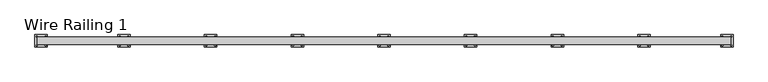
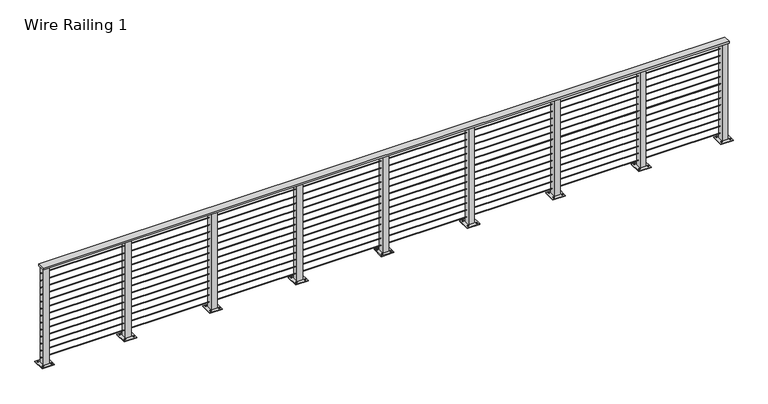
"""IFC4 building model written with IfcOpenShell, lengths in millimetres: railing geometry, Wire Railing 1."""

from ifc_helpers import new_model, si_unit, point, frame, frame_2d, origin, place, context, project, spatial, polyline, circle_curve, trimmed, segment, composite_curve, outline, extrude, source, transform, mapped, element, save


def wire_railing_1_4a66abef(model_context):
    return source(origin(), model_context, "Body", "SweptSolid", [
        extrude(outline(polyline([(-9024.2668771, -3185.4818735), (-9024.2668771, -3109.2818735), (-2001.1668771, -3109.2818735), (-2001.1668771, -3185.4818735), (-9024.2668771, -3185.4818735)])), frame((0.0, 0.0, 4502.15), z_axis=(0.0, 0.0, 1.0), x_axis=(1.0, 0.0, 0.0)), (0.0, 0.0, 1.0), 19.05),
        extrude(outline(composite_curve([segment(trimmed(circle_curve(frame_2d((-3147.3818735, 4442.61875)), 2.38125), [point((-3149.7631235, 4442.61875))], [point((-3145.0006235, 4442.61875))], False, "CARTESIAN"), True, "CONTINUOUS"), segment(trimmed(circle_curve(frame_2d((-3147.3818735, 4442.61875)), 2.38125), [point((-3145.0006235, 4442.61875))], [point((-3149.7631235, 4442.61875))], False, "CARTESIAN"), True, "CONTINUOUS")], self_intersect=False)), frame((-9024.2668771, 0.0, 0.0), z_axis=(1.0, 0.0, 0.0), x_axis=(0.0, 1.0, 0.0)), (0.0, 0.0, 1.0), 7023.1),
        extrude(outline(composite_curve([segment(trimmed(circle_curve(frame_2d((-3147.3818735, 4366.41875)), 2.38125), [point((-3149.7631235, 4366.41875))], [point((-3145.0006235, 4366.41875))], False, "CARTESIAN"), True, "CONTINUOUS"), segment(trimmed(circle_curve(frame_2d((-3147.3818735, 4366.41875)), 2.38125), [point((-3145.0006235, 4366.41875))], [point((-3149.7631235, 4366.41875))], False, "CARTESIAN"), True, "CONTINUOUS")], self_intersect=False)), frame((-9024.2668771, 0.0, 0.0), z_axis=(1.0, 0.0, 0.0), x_axis=(0.0, 1.0, 0.0)), (0.0, 0.0, 1.0), 7023.1),
        extrude(outline(composite_curve([segment(trimmed(circle_curve(frame_2d((-3147.3818735, 4290.21875)), 2.38125), [point((-3149.7631235, 4290.21875))], [point((-3145.0006235, 4290.21875))], False, "CARTESIAN"), True, "CONTINUOUS"), segment(trimmed(circle_curve(frame_2d((-3147.3818735, 4290.21875)), 2.38125), [point((-3145.0006235, 4290.21875))], [point((-3149.7631235, 4290.21875))], False, "CARTESIAN"), True, "CONTINUOUS")], self_intersect=False)), frame((-9024.2668771, 0.0, 0.0), z_axis=(1.0, 0.0, 0.0), x_axis=(0.0, 1.0, 0.0)), (0.0, 0.0, 1.0), 7023.1),
        extrude(outline(composite_curve([segment(trimmed(circle_curve(frame_2d((-3147.3818735, 4214.01875)), 2.38125), [point((-3149.7631235, 4214.01875))], [point((-3145.0006235, 4214.01875))], False, "CARTESIAN"), True, "CONTINUOUS"), segment(trimmed(circle_curve(frame_2d((-3147.3818735, 4214.01875)), 2.38125), [point((-3145.0006235, 4214.01875))], [point((-3149.7631235, 4214.01875))], False, "CARTESIAN"), True, "CONTINUOUS")], self_intersect=False)), frame((-9024.2668771, 0.0, 0.0), z_axis=(1.0, 0.0, 0.0), x_axis=(0.0, 1.0, 0.0)), (0.0, 0.0, 1.0), 7023.1),
        extrude(outline(composite_curve([segment(trimmed(circle_curve(frame_2d((-3147.3818735, 4137.81875)), 2.38125), [point((-3149.7631235, 4137.81875))], [point((-3145.0006235, 4137.81875))], False, "CARTESIAN"), True, "CONTINUOUS"), segment(trimmed(circle_curve(frame_2d((-3147.3818735, 4137.81875)), 2.38125), [point((-3145.0006235, 4137.81875))], [point((-3149.7631235, 4137.81875))], False, "CARTESIAN"), True, "CONTINUOUS")], self_intersect=False)), frame((-9024.2668771, 0.0, 0.0), z_axis=(1.0, 0.0, 0.0), x_axis=(0.0, 1.0, 0.0)), (0.0, 0.0, 1.0), 7023.1),
        extrude(outline(composite_curve([segment(trimmed(circle_curve(frame_2d((-3147.3818735, 4061.61875)), 2.38125), [point((-3149.7631235, 4061.61875))], [point((-3145.0006235, 4061.61875))], False, "CARTESIAN"), True, "CONTINUOUS"), segment(trimmed(circle_curve(frame_2d((-3147.3818735, 4061.61875)), 2.38125), [point((-3145.0006235, 4061.61875))], [point((-3149.7631235, 4061.61875))], False, "CARTESIAN"), True, "CONTINUOUS")], self_intersect=False)), frame((-9024.2668771, 0.0, 0.0), z_axis=(1.0, 0.0, 0.0), x_axis=(0.0, 1.0, 0.0)), (0.0, 0.0, 1.0), 7023.1),
        extrude(outline(composite_curve([segment(trimmed(circle_curve(frame_2d((-3147.3818735, 3985.41875)), 2.38125), [point((-3149.7631235, 3985.41875))], [point((-3145.0006235, 3985.41875))], False, "CARTESIAN"), True, "CONTINUOUS"), segment(trimmed(circle_curve(frame_2d((-3147.3818735, 3985.41875)), 2.38125), [point((-3145.0006235, 3985.41875))], [point((-3149.7631235, 3985.41875))], False, "CARTESIAN"), True, "CONTINUOUS")], self_intersect=False)), frame((-9024.2668771, 0.0, 0.0), z_axis=(1.0, 0.0, 0.0), x_axis=(0.0, 1.0, 0.0)), (0.0, 0.0, 1.0), 7023.1),
        extrude(outline(composite_curve([segment(trimmed(circle_curve(frame_2d((-3147.3818735, 3909.21875)), 2.38125), [point((-3149.7631235, 3909.21875))], [point((-3145.0006235, 3909.21875))], False, "CARTESIAN"), True, "CONTINUOUS"), segment(trimmed(circle_curve(frame_2d((-3147.3818735, 3909.21875)), 2.38125), [point((-3145.0006235, 3909.21875))], [point((-3149.7631235, 3909.21875))], False, "CARTESIAN"), True, "CONTINUOUS")], self_intersect=False)), frame((-9024.2668771, 0.0, 0.0), z_axis=(1.0, 0.0, 0.0), x_axis=(0.0, 1.0, 0.0)), (0.0, 0.0, 1.0), 7023.1),
        extrude(outline(composite_curve([segment(trimmed(circle_curve(frame_2d((-3147.3818735, 3833.01875)), 2.38125), [point((-3149.7631235, 3833.01875))], [point((-3145.0006235, 3833.01875))], False, "CARTESIAN"), True, "CONTINUOUS"), segment(trimmed(circle_curve(frame_2d((-3147.3818735, 3833.01875)), 2.38125), [point((-3145.0006235, 3833.01875))], [point((-3149.7631235, 3833.01875))], False, "CARTESIAN"), True, "CONTINUOUS")], self_intersect=False)), frame((-9024.2668771, 0.0, 0.0), z_axis=(1.0, 0.0, 0.0), x_axis=(0.0, 1.0, 0.0)), (0.0, 0.0, 1.0), 7023.1),
        extrude(outline(composite_curve([segment(trimmed(circle_curve(frame_2d((-3147.3818735, 3756.81875)), 2.38125), [point((-3149.7631235, 3756.81875))], [point((-3145.0006235, 3756.81875))], False, "CARTESIAN"), True, "CONTINUOUS"), segment(trimmed(circle_curve(frame_2d((-3147.3818735, 3756.81875)), 2.38125), [point((-3145.0006235, 3756.81875))], [point((-3149.7631235, 3756.81875))], False, "CARTESIAN"), True, "CONTINUOUS")], self_intersect=False)), frame((-9024.2668771, 0.0, 0.0), z_axis=(1.0, 0.0, 0.0), x_axis=(0.0, 1.0, 0.0)), (0.0, 0.0, 1.0), 7023.1),
        extrude(outline(composite_curve([segment(trimmed(circle_curve(frame_2d((-3147.3818735, 3680.61875)), 2.38125), [point((-3149.7631235, 3680.61875))], [point((-3145.0006235, 3680.61875))], False, "CARTESIAN"), True, "CONTINUOUS"), segment(trimmed(circle_curve(frame_2d((-3147.3818735, 3680.61875)), 2.38125), [point((-3145.0006235, 3680.61875))], [point((-3149.7631235, 3680.61875))], False, "CARTESIAN"), True, "CONTINUOUS")], self_intersect=False)), frame((-9024.2668771, 0.0, 0.0), z_axis=(1.0, 0.0, 0.0), x_axis=(0.0, 1.0, 0.0)), (0.0, 0.0, 1.0), 7023.1),
        extrude(outline(composite_curve([segment(trimmed(circle_curve(frame_2d((-3147.3818735, 3604.41875)), 2.38125), [point((-3149.7631235, 3604.41875))], [point((-3145.0006235, 3604.41875))], False, "CARTESIAN"), True, "CONTINUOUS"), segment(trimmed(circle_curve(frame_2d((-3147.3818735, 3604.41875)), 2.38125), [point((-3145.0006235, 3604.41875))], [point((-3149.7631235, 3604.41875))], False, "CARTESIAN"), True, "CONTINUOUS")], self_intersect=False)), frame((-9024.2668771, 0.0, 0.0), z_axis=(1.0, 0.0, 0.0), x_axis=(0.0, 1.0, 0.0)), (0.0, 0.0, 1.0), 7023.1),
        extrude(outline(composite_curve([segment(trimmed(circle_curve(frame_2d((-3147.3818735, 3528.21875)), 2.38125), [point((-3149.7631235, 3528.21875))], [point((-3145.0006235, 3528.21875))], False, "CARTESIAN"), True, "CONTINUOUS"), segment(trimmed(circle_curve(frame_2d((-3147.3818735, 3528.21875)), 2.38125), [point((-3145.0006235, 3528.21875))], [point((-3149.7631235, 3528.21875))], False, "CARTESIAN"), True, "CONTINUOUS")], self_intersect=False)), frame((-9024.2668771, 0.0, 0.0), z_axis=(1.0, 0.0, 0.0), x_axis=(0.0, 1.0, 0.0)), (0.0, 0.0, 1.0), 7023.1),
        extrude(outline(composite_curve([segment(trimmed(circle_curve(frame_2d((-2923.5043771, -3102.9318735)), 6.35), [point((-2923.5043771, -3096.5818735))], [point((-2923.5043771, -3109.2818735))], False, "CARTESIAN"), True, "CONTINUOUS"), segment(trimmed(circle_curve(frame_2d((-2923.5043771, -3102.9318735)), 6.35), [point((-2923.5043771, -3109.2818735))], [point((-2923.5043771, -3096.5818735))], False, "CARTESIAN"), True, "CONTINUOUS")], self_intersect=False)), frame((0.0, 0.0, 3454.4), z_axis=(0.0, 0.0, 1.0), x_axis=(1.0, 0.0, 0.0)), (0.0, 0.0, 1.0), 12.7),
        extrude(outline(composite_curve([segment(trimmed(circle_curve(frame_2d((-2923.5043771, -3191.8318735)), 6.35), [point((-2923.5043771, -3185.4818735))], [point((-2923.5043771, -3198.1818735))], False, "CARTESIAN"), True, "CONTINUOUS"), segment(trimmed(circle_curve(frame_2d((-2923.5043771, -3191.8318735)), 6.35), [point((-2923.5043771, -3198.1818735))], [point((-2923.5043771, -3185.4818735))], False, "CARTESIAN"), True, "CONTINUOUS")], self_intersect=False)), frame((0.0, 0.0, 3454.4), z_axis=(0.0, 0.0, 1.0), x_axis=(1.0, 0.0, 0.0)), (0.0, 0.0, 1.0), 12.7),
        extrude(outline(composite_curve([segment(trimmed(circle_curve(frame_2d((-2834.6043771, -3102.9318735)), 6.35), [point((-2834.6043771, -3096.5818735))], [point((-2834.6043771, -3109.2818735))], False, "CARTESIAN"), True, "CONTINUOUS"), segment(trimmed(circle_curve(frame_2d((-2834.6043771, -3102.9318735)), 6.35), [point((-2834.6043771, -3109.2818735))], [point((-2834.6043771, -3096.5818735))], False, "CARTESIAN"), True, "CONTINUOUS")], self_intersect=False)), frame((0.0, 0.0, 3454.4), z_axis=(0.0, 0.0, 1.0), x_axis=(1.0, 0.0, 0.0)), (0.0, 0.0, 1.0), 12.7),
        extrude(outline(composite_curve([segment(trimmed(circle_curve(frame_2d((-2834.6043771, -3191.8318735)), 6.35), [point((-2834.6043771, -3185.4818735))], [point((-2834.6043771, -3198.1818735))], False, "CARTESIAN"), True, "CONTINUOUS"), segment(trimmed(circle_curve(frame_2d((-2834.6043771, -3191.8318735)), 6.35), [point((-2834.6043771, -3198.1818735))], [point((-2834.6043771, -3185.4818735))], False, "CARTESIAN"), True, "CONTINUOUS")], self_intersect=False)), frame((0.0, 0.0, 3454.4), z_axis=(0.0, 0.0, 1.0), x_axis=(1.0, 0.0, 0.0)), (0.0, 0.0, 1.0), 12.7),
        extrude(outline(polyline([(-2942.5543771, -3210.8818735), (-2942.5543771, -3083.8818735), (-2815.5543771, -3083.8818735), (-2815.5543771, -3210.8818735), (-2942.5543771, -3210.8818735)])), frame((0.0, 0.0, 3454.4), z_axis=(0.0, 0.0, 1.0), x_axis=(1.0, 0.0, 0.0)), (0.0, 0.0, 1.0), 6.35),
        extrude(outline(polyline([(-2909.2168771, -3177.5443735), (-2909.2168771, -3117.2193735), (-2848.8918771, -3117.2193735), (-2848.8918771, -3177.5443735), (-2909.2168771, -3177.5443735)]), holes=[polyline([(-2902.8668771, -3171.1943735), (-2855.2418771, -3171.1943735), (-2855.2418771, -3123.5693735), (-2902.8668771, -3123.5693735), (-2902.8668771, -3171.1943735)])]), frame((0.0, 0.0, 3454.4), z_axis=(0.0, 0.0, 1.0), x_axis=(1.0, 0.0, 0.0)), (0.0, 0.0, 1.0), 1047.75),
        extrude(outline(composite_curve([segment(trimmed(circle_curve(frame_2d((-3801.3918771, -3102.9318735)), 6.35), [point((-3801.3918771, -3096.5818735))], [point((-3801.3918771, -3109.2818735))], False, "CARTESIAN"), True, "CONTINUOUS"), segment(trimmed(circle_curve(frame_2d((-3801.3918771, -3102.9318735)), 6.35), [point((-3801.3918771, -3109.2818735))], [point((-3801.3918771, -3096.5818735))], False, "CARTESIAN"), True, "CONTINUOUS")], self_intersect=False)), frame((0.0, 0.0, 3454.4), z_axis=(0.0, 0.0, 1.0), x_axis=(1.0, 0.0, 0.0)), (0.0, 0.0, 1.0), 12.7),
        extrude(outline(composite_curve([segment(trimmed(circle_curve(frame_2d((-3801.3918771, -3191.8318735)), 6.35), [point((-3801.3918771, -3185.4818735))], [point((-3801.3918771, -3198.1818735))], False, "CARTESIAN"), True, "CONTINUOUS"), segment(trimmed(circle_curve(frame_2d((-3801.3918771, -3191.8318735)), 6.35), [point((-3801.3918771, -3198.1818735))], [point((-3801.3918771, -3185.4818735))], False, "CARTESIAN"), True, "CONTINUOUS")], self_intersect=False)), frame((0.0, 0.0, 3454.4), z_axis=(0.0, 0.0, 1.0), x_axis=(1.0, 0.0, 0.0)), (0.0, 0.0, 1.0), 12.7),
        extrude(outline(composite_curve([segment(trimmed(circle_curve(frame_2d((-3712.4918771, -3102.9318735)), 6.35), [point((-3712.4918771, -3096.5818735))], [point((-3712.4918771, -3109.2818735))], False, "CARTESIAN"), True, "CONTINUOUS"), segment(trimmed(circle_curve(frame_2d((-3712.4918771, -3102.9318735)), 6.35), [point((-3712.4918771, -3109.2818735))], [point((-3712.4918771, -3096.5818735))], False, "CARTESIAN"), True, "CONTINUOUS")], self_intersect=False)), frame((0.0, 0.0, 3454.4), z_axis=(0.0, 0.0, 1.0), x_axis=(1.0, 0.0, 0.0)), (0.0, 0.0, 1.0), 12.7),
        extrude(outline(composite_curve([segment(trimmed(circle_curve(frame_2d((-3712.4918771, -3191.8318735)), 6.35), [point((-3712.4918771, -3185.4818735))], [point((-3712.4918771, -3198.1818735))], False, "CARTESIAN"), True, "CONTINUOUS"), segment(trimmed(circle_curve(frame_2d((-3712.4918771, -3191.8318735)), 6.35), [point((-3712.4918771, -3198.1818735))], [point((-3712.4918771, -3185.4818735))], False, "CARTESIAN"), True, "CONTINUOUS")], self_intersect=False)), frame((0.0, 0.0, 3454.4), z_axis=(0.0, 0.0, 1.0), x_axis=(1.0, 0.0, 0.0)), (0.0, 0.0, 1.0), 12.7),
        extrude(outline(polyline([(-3820.4418771, -3210.8818735), (-3820.4418771, -3083.8818735), (-3693.4418771, -3083.8818735), (-3693.4418771, -3210.8818735), (-3820.4418771, -3210.8818735)])), frame((0.0, 0.0, 3454.4), z_axis=(0.0, 0.0, 1.0), x_axis=(1.0, 0.0, 0.0)), (0.0, 0.0, 1.0), 6.35),
        extrude(outline(polyline([(-3787.1043771, -3177.5443735), (-3787.1043771, -3117.2193735), (-3726.7793771, -3117.2193735), (-3726.7793771, -3177.5443735), (-3787.1043771, -3177.5443735)]), holes=[polyline([(-3780.7543771, -3171.1943735), (-3733.1293771, -3171.1943735), (-3733.1293771, -3123.5693735), (-3780.7543771, -3123.5693735), (-3780.7543771, -3171.1943735)])]), frame((0.0, 0.0, 3454.4), z_axis=(0.0, 0.0, 1.0), x_axis=(1.0, 0.0, 0.0)), (0.0, 0.0, 1.0), 1047.75),
        extrude(outline(composite_curve([segment(trimmed(circle_curve(frame_2d((-4679.2793771, -3102.9318735)), 6.35), [point((-4679.2793771, -3096.5818735))], [point((-4679.2793771, -3109.2818735))], False, "CARTESIAN"), True, "CONTINUOUS"), segment(trimmed(circle_curve(frame_2d((-4679.2793771, -3102.9318735)), 6.35), [point((-4679.2793771, -3109.2818735))], [point((-4679.2793771, -3096.5818735))], False, "CARTESIAN"), True, "CONTINUOUS")], self_intersect=False)), frame((0.0, 0.0, 3454.4), z_axis=(0.0, 0.0, 1.0), x_axis=(1.0, 0.0, 0.0)), (0.0, 0.0, 1.0), 12.7),
        extrude(outline(composite_curve([segment(trimmed(circle_curve(frame_2d((-4679.2793771, -3191.8318735)), 6.35), [point((-4679.2793771, -3185.4818735))], [point((-4679.2793771, -3198.1818735))], False, "CARTESIAN"), True, "CONTINUOUS"), segment(trimmed(circle_curve(frame_2d((-4679.2793771, -3191.8318735)), 6.35), [point((-4679.2793771, -3198.1818735))], [point((-4679.2793771, -3185.4818735))], False, "CARTESIAN"), True, "CONTINUOUS")], self_intersect=False)), frame((0.0, 0.0, 3454.4), z_axis=(0.0, 0.0, 1.0), x_axis=(1.0, 0.0, 0.0)), (0.0, 0.0, 1.0), 12.7),
        extrude(outline(composite_curve([segment(trimmed(circle_curve(frame_2d((-4590.3793771, -3102.9318735)), 6.35), [point((-4590.3793771, -3096.5818735))], [point((-4590.3793771, -3109.2818735))], False, "CARTESIAN"), True, "CONTINUOUS"), segment(trimmed(circle_curve(frame_2d((-4590.3793771, -3102.9318735)), 6.35), [point((-4590.3793771, -3109.2818735))], [point((-4590.3793771, -3096.5818735))], False, "CARTESIAN"), True, "CONTINUOUS")], self_intersect=False)), frame((0.0, 0.0, 3454.4), z_axis=(0.0, 0.0, 1.0), x_axis=(1.0, 0.0, 0.0)), (0.0, 0.0, 1.0), 12.7),
        extrude(outline(composite_curve([segment(trimmed(circle_curve(frame_2d((-4590.3793771, -3191.8318735)), 6.35), [point((-4590.3793771, -3185.4818735))], [point((-4590.3793771, -3198.1818735))], False, "CARTESIAN"), True, "CONTINUOUS"), segment(trimmed(circle_curve(frame_2d((-4590.3793771, -3191.8318735)), 6.35), [point((-4590.3793771, -3198.1818735))], [point((-4590.3793771, -3185.4818735))], False, "CARTESIAN"), True, "CONTINUOUS")], self_intersect=False)), frame((0.0, 0.0, 3454.4), z_axis=(0.0, 0.0, 1.0), x_axis=(1.0, 0.0, 0.0)), (0.0, 0.0, 1.0), 12.7),
        extrude(outline(polyline([(-4698.3293771, -3210.8818735), (-4698.3293771, -3083.8818735), (-4571.3293771, -3083.8818735), (-4571.3293771, -3210.8818735), (-4698.3293771, -3210.8818735)])), frame((0.0, 0.0, 3454.4), z_axis=(0.0, 0.0, 1.0), x_axis=(1.0, 0.0, 0.0)), (0.0, 0.0, 1.0), 6.35),
        extrude(outline(polyline([(-4664.9918771, -3177.5443735), (-4664.9918771, -3117.2193735), (-4604.6668771, -3117.2193735), (-4604.6668771, -3177.5443735), (-4664.9918771, -3177.5443735)]), holes=[polyline([(-4658.6418771, -3171.1943735), (-4611.0168771, -3171.1943735), (-4611.0168771, -3123.5693735), (-4658.6418771, -3123.5693735), (-4658.6418771, -3171.1943735)])]), frame((0.0, 0.0, 3454.4), z_axis=(0.0, 0.0, 1.0), x_axis=(1.0, 0.0, 0.0)), (0.0, 0.0, 1.0), 1047.75),
        extrude(outline(composite_curve([segment(trimmed(circle_curve(frame_2d((-5557.1668771, -3102.9318735)), 6.35), [point((-5557.1668771, -3096.5818735))], [point((-5557.1668771, -3109.2818735))], False, "CARTESIAN"), True, "CONTINUOUS"), segment(trimmed(circle_curve(frame_2d((-5557.1668771, -3102.9318735)), 6.35), [point((-5557.1668771, -3109.2818735))], [point((-5557.1668771, -3096.5818735))], False, "CARTESIAN"), True, "CONTINUOUS")], self_intersect=False)), frame((0.0, 0.0, 3454.4), z_axis=(0.0, 0.0, 1.0), x_axis=(1.0, 0.0, 0.0)), (0.0, 0.0, 1.0), 12.7),
        extrude(outline(composite_curve([segment(trimmed(circle_curve(frame_2d((-5557.1668771, -3191.8318735)), 6.35), [point((-5557.1668771, -3185.4818735))], [point((-5557.1668771, -3198.1818735))], False, "CARTESIAN"), True, "CONTINUOUS"), segment(trimmed(circle_curve(frame_2d((-5557.1668771, -3191.8318735)), 6.35), [point((-5557.1668771, -3198.1818735))], [point((-5557.1668771, -3185.4818735))], False, "CARTESIAN"), True, "CONTINUOUS")], self_intersect=False)), frame((0.0, 0.0, 3454.4), z_axis=(0.0, 0.0, 1.0), x_axis=(1.0, 0.0, 0.0)), (0.0, 0.0, 1.0), 12.7),
        extrude(outline(composite_curve([segment(trimmed(circle_curve(frame_2d((-5468.2668771, -3102.9318735)), 6.35), [point((-5468.2668771, -3096.5818735))], [point((-5468.2668771, -3109.2818735))], False, "CARTESIAN"), True, "CONTINUOUS"), segment(trimmed(circle_curve(frame_2d((-5468.2668771, -3102.9318735)), 6.35), [point((-5468.2668771, -3109.2818735))], [point((-5468.2668771, -3096.5818735))], False, "CARTESIAN"), True, "CONTINUOUS")], self_intersect=False)), frame((0.0, 0.0, 3454.4), z_axis=(0.0, 0.0, 1.0), x_axis=(1.0, 0.0, 0.0)), (0.0, 0.0, 1.0), 12.7),
        extrude(outline(composite_curve([segment(trimmed(circle_curve(frame_2d((-5468.2668771, -3191.8318735)), 6.35), [point((-5468.2668771, -3185.4818735))], [point((-5468.2668771, -3198.1818735))], False, "CARTESIAN"), True, "CONTINUOUS"), segment(trimmed(circle_curve(frame_2d((-5468.2668771, -3191.8318735)), 6.35), [point((-5468.2668771, -3198.1818735))], [point((-5468.2668771, -3185.4818735))], False, "CARTESIAN"), True, "CONTINUOUS")], self_intersect=False)), frame((0.0, 0.0, 3454.4), z_axis=(0.0, 0.0, 1.0), x_axis=(1.0, 0.0, 0.0)), (0.0, 0.0, 1.0), 12.7),
        extrude(outline(polyline([(-5576.2168771, -3210.8818735), (-5576.2168771, -3083.8818735), (-5449.2168771, -3083.8818735), (-5449.2168771, -3210.8818735), (-5576.2168771, -3210.8818735)])), frame((0.0, 0.0, 3454.4), z_axis=(0.0, 0.0, 1.0), x_axis=(1.0, 0.0, 0.0)), (0.0, 0.0, 1.0), 6.35),
        extrude(outline(polyline([(-5542.8793771, -3177.5443735), (-5542.8793771, -3117.2193735), (-5482.5543771, -3117.2193735), (-5482.5543771, -3177.5443735), (-5542.8793771, -3177.5443735)]), holes=[polyline([(-5536.5293771, -3171.1943735), (-5488.9043771, -3171.1943735), (-5488.9043771, -3123.5693735), (-5536.5293771, -3123.5693735), (-5536.5293771, -3171.1943735)])]), frame((0.0, 0.0, 3454.4), z_axis=(0.0, 0.0, 1.0), x_axis=(1.0, 0.0, 0.0)), (0.0, 0.0, 1.0), 1047.75),
        extrude(outline(composite_curve([segment(trimmed(circle_curve(frame_2d((-6435.0543771, -3102.9318735)), 6.35), [point((-6435.0543771, -3096.5818735))], [point((-6435.0543771, -3109.2818735))], False, "CARTESIAN"), True, "CONTINUOUS"), segment(trimmed(circle_curve(frame_2d((-6435.0543771, -3102.9318735)), 6.35), [point((-6435.0543771, -3109.2818735))], [point((-6435.0543771, -3096.5818735))], False, "CARTESIAN"), True, "CONTINUOUS")], self_intersect=False)), frame((0.0, 0.0, 3454.4), z_axis=(0.0, 0.0, 1.0), x_axis=(1.0, 0.0, 0.0)), (0.0, 0.0, 1.0), 12.7),
        extrude(outline(composite_curve([segment(trimmed(circle_curve(frame_2d((-6435.0543771, -3191.8318735)), 6.35), [point((-6435.0543771, -3185.4818735))], [point((-6435.0543771, -3198.1818735))], False, "CARTESIAN"), True, "CONTINUOUS"), segment(trimmed(circle_curve(frame_2d((-6435.0543771, -3191.8318735)), 6.35), [point((-6435.0543771, -3198.1818735))], [point((-6435.0543771, -3185.4818735))], False, "CARTESIAN"), True, "CONTINUOUS")], self_intersect=False)), frame((0.0, 0.0, 3454.4), z_axis=(0.0, 0.0, 1.0), x_axis=(1.0, 0.0, 0.0)), (0.0, 0.0, 1.0), 12.7),
        extrude(outline(composite_curve([segment(trimmed(circle_curve(frame_2d((-6346.1543771, -3102.9318735)), 6.35), [point((-6346.1543771, -3096.5818735))], [point((-6346.1543771, -3109.2818735))], False, "CARTESIAN"), True, "CONTINUOUS"), segment(trimmed(circle_curve(frame_2d((-6346.1543771, -3102.9318735)), 6.35), [point((-6346.1543771, -3109.2818735))], [point((-6346.1543771, -3096.5818735))], False, "CARTESIAN"), True, "CONTINUOUS")], self_intersect=False)), frame((0.0, 0.0, 3454.4), z_axis=(0.0, 0.0, 1.0), x_axis=(1.0, 0.0, 0.0)), (0.0, 0.0, 1.0), 12.7),
        extrude(outline(composite_curve([segment(trimmed(circle_curve(frame_2d((-6346.1543771, -3191.8318735)), 6.35), [point((-6346.1543771, -3185.4818735))], [point((-6346.1543771, -3198.1818735))], False, "CARTESIAN"), True, "CONTINUOUS"), segment(trimmed(circle_curve(frame_2d((-6346.1543771, -3191.8318735)), 6.35), [point((-6346.1543771, -3198.1818735))], [point((-6346.1543771, -3185.4818735))], False, "CARTESIAN"), True, "CONTINUOUS")], self_intersect=False)), frame((0.0, 0.0, 3454.4), z_axis=(0.0, 0.0, 1.0), x_axis=(1.0, 0.0, 0.0)), (0.0, 0.0, 1.0), 12.7),
        extrude(outline(polyline([(-6454.1043771, -3210.8818735), (-6454.1043771, -3083.8818735), (-6327.1043771, -3083.8818735), (-6327.1043771, -3210.8818735), (-6454.1043771, -3210.8818735)])), frame((0.0, 0.0, 3454.4), z_axis=(0.0, 0.0, 1.0), x_axis=(1.0, 0.0, 0.0)), (0.0, 0.0, 1.0), 6.35),
        extrude(outline(polyline([(-6420.7668771, -3177.5443735), (-6420.7668771, -3117.2193735), (-6360.4418771, -3117.2193735), (-6360.4418771, -3177.5443735), (-6420.7668771, -3177.5443735)]), holes=[polyline([(-6414.4168771, -3171.1943735), (-6366.7918771, -3171.1943735), (-6366.7918771, -3123.5693735), (-6414.4168771, -3123.5693735), (-6414.4168771, -3171.1943735)])]), frame((0.0, 0.0, 3454.4), z_axis=(0.0, 0.0, 1.0), x_axis=(1.0, 0.0, 0.0)), (0.0, 0.0, 1.0), 1047.75),
        extrude(outline(composite_curve([segment(trimmed(circle_curve(frame_2d((-7312.9418771, -3102.9318735)), 6.35), [point((-7312.9418771, -3096.5818735))], [point((-7312.9418771, -3109.2818735))], False, "CARTESIAN"), True, "CONTINUOUS"), segment(trimmed(circle_curve(frame_2d((-7312.9418771, -3102.9318735)), 6.35), [point((-7312.9418771, -3109.2818735))], [point((-7312.9418771, -3096.5818735))], False, "CARTESIAN"), True, "CONTINUOUS")], self_intersect=False)), frame((0.0, 0.0, 3454.4), z_axis=(0.0, 0.0, 1.0), x_axis=(1.0, 0.0, 0.0)), (0.0, 0.0, 1.0), 12.7),
        extrude(outline(composite_curve([segment(trimmed(circle_curve(frame_2d((-7312.9418771, -3191.8318735)), 6.35), [point((-7312.9418771, -3185.4818735))], [point((-7312.9418771, -3198.1818735))], False, "CARTESIAN"), True, "CONTINUOUS"), segment(trimmed(circle_curve(frame_2d((-7312.9418771, -3191.8318735)), 6.35), [point((-7312.9418771, -3198.1818735))], [point((-7312.9418771, -3185.4818735))], False, "CARTESIAN"), True, "CONTINUOUS")], self_intersect=False)), frame((0.0, 0.0, 3454.4), z_axis=(0.0, 0.0, 1.0), x_axis=(1.0, 0.0, 0.0)), (0.0, 0.0, 1.0), 12.7),
        extrude(outline(composite_curve([segment(trimmed(circle_curve(frame_2d((-7224.0418771, -3102.9318735)), 6.35), [point((-7224.0418771, -3096.5818735))], [point((-7224.0418771, -3109.2818735))], False, "CARTESIAN"), True, "CONTINUOUS"), segment(trimmed(circle_curve(frame_2d((-7224.0418771, -3102.9318735)), 6.35), [point((-7224.0418771, -3109.2818735))], [point((-7224.0418771, -3096.5818735))], False, "CARTESIAN"), True, "CONTINUOUS")], self_intersect=False)), frame((0.0, 0.0, 3454.4), z_axis=(0.0, 0.0, 1.0), x_axis=(1.0, 0.0, 0.0)), (0.0, 0.0, 1.0), 12.7),
        extrude(outline(composite_curve([segment(trimmed(circle_curve(frame_2d((-7224.0418771, -3191.8318735)), 6.35), [point((-7224.0418771, -3185.4818735))], [point((-7224.0418771, -3198.1818735))], False, "CARTESIAN"), True, "CONTINUOUS"), segment(trimmed(circle_curve(frame_2d((-7224.0418771, -3191.8318735)), 6.35), [point((-7224.0418771, -3198.1818735))], [point((-7224.0418771, -3185.4818735))], False, "CARTESIAN"), True, "CONTINUOUS")], self_intersect=False)), frame((0.0, 0.0, 3454.4), z_axis=(0.0, 0.0, 1.0), x_axis=(1.0, 0.0, 0.0)), (0.0, 0.0, 1.0), 12.7),
        extrude(outline(polyline([(-7331.9918771, -3210.8818735), (-7331.9918771, -3083.8818735), (-7204.9918771, -3083.8818735), (-7204.9918771, -3210.8818735), (-7331.9918771, -3210.8818735)])), frame((0.0, 0.0, 3454.4), z_axis=(0.0, 0.0, 1.0), x_axis=(1.0, 0.0, 0.0)), (0.0, 0.0, 1.0), 6.35),
        extrude(outline(polyline([(-7298.6543771, -3177.5443735), (-7298.6543771, -3117.2193735), (-7238.3293771, -3117.2193735), (-7238.3293771, -3177.5443735), (-7298.6543771, -3177.5443735)]), holes=[polyline([(-7292.3043771, -3171.1943735), (-7244.6793771, -3171.1943735), (-7244.6793771, -3123.5693735), (-7292.3043771, -3123.5693735), (-7292.3043771, -3171.1943735)])]), frame((0.0, 0.0, 3454.4), z_axis=(0.0, 0.0, 1.0), x_axis=(1.0, 0.0, 0.0)), (0.0, 0.0, 1.0), 1047.75),
        extrude(outline(composite_curve([segment(trimmed(circle_curve(frame_2d((-8190.8293771, -3102.9318735)), 6.35), [point((-8190.8293771, -3096.5818735))], [point((-8190.8293771, -3109.2818735))], False, "CARTESIAN"), True, "CONTINUOUS"), segment(trimmed(circle_curve(frame_2d((-8190.8293771, -3102.9318735)), 6.35), [point((-8190.8293771, -3109.2818735))], [point((-8190.8293771, -3096.5818735))], False, "CARTESIAN"), True, "CONTINUOUS")], self_intersect=False)), frame((0.0, 0.0, 3454.4), z_axis=(0.0, 0.0, 1.0), x_axis=(1.0, 0.0, 0.0)), (0.0, 0.0, 1.0), 12.7),
        extrude(outline(composite_curve([segment(trimmed(circle_curve(frame_2d((-8190.8293771, -3191.8318735)), 6.35), [point((-8190.8293771, -3185.4818735))], [point((-8190.8293771, -3198.1818735))], False, "CARTESIAN"), True, "CONTINUOUS"), segment(trimmed(circle_curve(frame_2d((-8190.8293771, -3191.8318735)), 6.35), [point((-8190.8293771, -3198.1818735))], [point((-8190.8293771, -3185.4818735))], False, "CARTESIAN"), True, "CONTINUOUS")], self_intersect=False)), frame((0.0, 0.0, 3454.4), z_axis=(0.0, 0.0, 1.0), x_axis=(1.0, 0.0, 0.0)), (0.0, 0.0, 1.0), 12.7),
        extrude(outline(composite_curve([segment(trimmed(circle_curve(frame_2d((-8101.9293771, -3102.9318735)), 6.35), [point((-8101.9293771, -3096.5818735))], [point((-8101.9293771, -3109.2818735))], False, "CARTESIAN"), True, "CONTINUOUS"), segment(trimmed(circle_curve(frame_2d((-8101.9293771, -3102.9318735)), 6.35), [point((-8101.9293771, -3109.2818735))], [point((-8101.9293771, -3096.5818735))], False, "CARTESIAN"), True, "CONTINUOUS")], self_intersect=False)), frame((0.0, 0.0, 3454.4), z_axis=(0.0, 0.0, 1.0), x_axis=(1.0, 0.0, 0.0)), (0.0, 0.0, 1.0), 12.7),
        extrude(outline(composite_curve([segment(trimmed(circle_curve(frame_2d((-8101.9293771, -3191.8318735)), 6.35), [point((-8101.9293771, -3185.4818735))], [point((-8101.9293771, -3198.1818735))], False, "CARTESIAN"), True, "CONTINUOUS"), segment(trimmed(circle_curve(frame_2d((-8101.9293771, -3191.8318735)), 6.35), [point((-8101.9293771, -3198.1818735))], [point((-8101.9293771, -3185.4818735))], False, "CARTESIAN"), True, "CONTINUOUS")], self_intersect=False)), frame((0.0, 0.0, 3454.4), z_axis=(0.0, 0.0, 1.0), x_axis=(1.0, 0.0, 0.0)), (0.0, 0.0, 1.0), 12.7),
        extrude(outline(polyline([(-8209.8793771, -3210.8818735), (-8209.8793771, -3083.8818735), (-8082.8793771, -3083.8818735), (-8082.8793771, -3210.8818735), (-8209.8793771, -3210.8818735)])), frame((0.0, 0.0, 3454.4), z_axis=(0.0, 0.0, 1.0), x_axis=(1.0, 0.0, 0.0)), (0.0, 0.0, 1.0), 6.35),
        extrude(outline(polyline([(-8176.5418771, -3177.5443735), (-8176.5418771, -3117.2193735), (-8116.2168771, -3117.2193735), (-8116.2168771, -3177.5443735), (-8176.5418771, -3177.5443735)]), holes=[polyline([(-8170.1918771, -3171.1943735), (-8122.5668771, -3171.1943735), (-8122.5668771, -3123.5693735), (-8170.1918771, -3123.5693735), (-8170.1918771, -3171.1943735)])]), frame((0.0, 0.0, 3454.4), z_axis=(0.0, 0.0, 1.0), x_axis=(1.0, 0.0, 0.0)), (0.0, 0.0, 1.0), 1047.75),
        extrude(outline(composite_curve([segment(trimmed(circle_curve(frame_2d((-2083.7168771, -3102.9318735)), 6.35), [point((-2083.7168771, -3096.5818735))], [point((-2083.7168771, -3109.2818735))], False, "CARTESIAN"), True, "CONTINUOUS"), segment(trimmed(circle_curve(frame_2d((-2083.7168771, -3102.9318735)), 6.35), [point((-2083.7168771, -3109.2818735))], [point((-2083.7168771, -3096.5818735))], False, "CARTESIAN"), True, "CONTINUOUS")], self_intersect=False)), frame((0.0, 0.0, 3454.4), z_axis=(0.0, 0.0, 1.0), x_axis=(1.0, 0.0, 0.0)), (0.0, 0.0, 1.0), 12.7),
        extrude(outline(composite_curve([segment(trimmed(circle_curve(frame_2d((-2083.7168771, -3191.8318735)), 6.35), [point((-2083.7168771, -3185.4818735))], [point((-2083.7168771, -3198.1818735))], False, "CARTESIAN"), True, "CONTINUOUS"), segment(trimmed(circle_curve(frame_2d((-2083.7168771, -3191.8318735)), 6.35), [point((-2083.7168771, -3198.1818735))], [point((-2083.7168771, -3185.4818735))], False, "CARTESIAN"), True, "CONTINUOUS")], self_intersect=False)), frame((0.0, 0.0, 3454.4), z_axis=(0.0, 0.0, 1.0), x_axis=(1.0, 0.0, 0.0)), (0.0, 0.0, 1.0), 12.7),
        extrude(outline(composite_curve([segment(trimmed(circle_curve(frame_2d((-1994.8168771, -3102.9318735)), 6.35), [point((-1994.8168771, -3096.5818735))], [point((-1994.8168771, -3109.2818735))], False, "CARTESIAN"), True, "CONTINUOUS"), segment(trimmed(circle_curve(frame_2d((-1994.8168771, -3102.9318735)), 6.35), [point((-1994.8168771, -3109.2818735))], [point((-1994.8168771, -3096.5818735))], False, "CARTESIAN"), True, "CONTINUOUS")], self_intersect=False)), frame((0.0, 0.0, 3454.4), z_axis=(0.0, 0.0, 1.0), x_axis=(1.0, 0.0, 0.0)), (0.0, 0.0, 1.0), 12.7),
        extrude(outline(composite_curve([segment(trimmed(circle_curve(frame_2d((-1994.8168771, -3191.8318735)), 6.35), [point((-1994.8168771, -3185.4818735))], [point((-1994.8168771, -3198.1818735))], False, "CARTESIAN"), True, "CONTINUOUS"), segment(trimmed(circle_curve(frame_2d((-1994.8168771, -3191.8318735)), 6.35), [point((-1994.8168771, -3198.1818735))], [point((-1994.8168771, -3185.4818735))], False, "CARTESIAN"), True, "CONTINUOUS")], self_intersect=False)), frame((0.0, 0.0, 3454.4), z_axis=(0.0, 0.0, 1.0), x_axis=(1.0, 0.0, 0.0)), (0.0, 0.0, 1.0), 12.7),
        extrude(outline(polyline([(-2102.7668771, -3210.8818735), (-2102.7668771, -3083.8818735), (-1975.7668771, -3083.8818735), (-1975.7668771, -3210.8818735), (-2102.7668771, -3210.8818735)])), frame((0.0, 0.0, 3454.4), z_axis=(0.0, 0.0, 1.0), x_axis=(1.0, 0.0, 0.0)), (0.0, 0.0, 1.0), 6.35),
        extrude(outline(polyline([(-2069.4293771, -3177.5443735), (-2069.4293771, -3117.2193735), (-2009.1043771, -3117.2193735), (-2009.1043771, -3177.5443735), (-2069.4293771, -3177.5443735)]), holes=[polyline([(-2063.0793771, -3171.1943735), (-2015.4543771, -3171.1943735), (-2015.4543771, -3123.5693735), (-2063.0793771, -3123.5693735), (-2063.0793771, -3171.1943735)])]), frame((0.0, 0.0, 3454.4), z_axis=(0.0, 0.0, 1.0), x_axis=(1.0, 0.0, 0.0)), (0.0, 0.0, 1.0), 1047.75),
        extrude(outline(composite_curve([segment(trimmed(circle_curve(frame_2d((-9030.6168771, -3102.9318735)), 6.35), [point((-9030.6168771, -3096.5818735))], [point((-9030.6168771, -3109.2818735))], False, "CARTESIAN"), True, "CONTINUOUS"), segment(trimmed(circle_curve(frame_2d((-9030.6168771, -3102.9318735)), 6.35), [point((-9030.6168771, -3109.2818735))], [point((-9030.6168771, -3096.5818735))], False, "CARTESIAN"), True, "CONTINUOUS")], self_intersect=False)), frame((0.0, 0.0, 3454.4), z_axis=(0.0, 0.0, 1.0), x_axis=(1.0, 0.0, 0.0)), (0.0, 0.0, 1.0), 12.7),
        extrude(outline(composite_curve([segment(trimmed(circle_curve(frame_2d((-9030.6168771, -3191.8318735)), 6.35), [point((-9030.6168771, -3185.4818735))], [point((-9030.6168771, -3198.1818735))], False, "CARTESIAN"), True, "CONTINUOUS"), segment(trimmed(circle_curve(frame_2d((-9030.6168771, -3191.8318735)), 6.35), [point((-9030.6168771, -3198.1818735))], [point((-9030.6168771, -3185.4818735))], False, "CARTESIAN"), True, "CONTINUOUS")], self_intersect=False)), frame((0.0, 0.0, 3454.4), z_axis=(0.0, 0.0, 1.0), x_axis=(1.0, 0.0, 0.0)), (0.0, 0.0, 1.0), 12.7),
        extrude(outline(composite_curve([segment(trimmed(circle_curve(frame_2d((-8941.7168771, -3102.9318735)), 6.35), [point((-8941.7168771, -3096.5818735))], [point((-8941.7168771, -3109.2818735))], False, "CARTESIAN"), True, "CONTINUOUS"), segment(trimmed(circle_curve(frame_2d((-8941.7168771, -3102.9318735)), 6.35), [point((-8941.7168771, -3109.2818735))], [point((-8941.7168771, -3096.5818735))], False, "CARTESIAN"), True, "CONTINUOUS")], self_intersect=False)), frame((0.0, 0.0, 3454.4), z_axis=(0.0, 0.0, 1.0), x_axis=(1.0, 0.0, 0.0)), (0.0, 0.0, 1.0), 12.7),
        extrude(outline(composite_curve([segment(trimmed(circle_curve(frame_2d((-8941.7168771, -3191.8318735)), 6.35), [point((-8941.7168771, -3185.4818735))], [point((-8941.7168771, -3198.1818735))], False, "CARTESIAN"), True, "CONTINUOUS"), segment(trimmed(circle_curve(frame_2d((-8941.7168771, -3191.8318735)), 6.35), [point((-8941.7168771, -3198.1818735))], [point((-8941.7168771, -3185.4818735))], False, "CARTESIAN"), True, "CONTINUOUS")], self_intersect=False)), frame((0.0, 0.0, 3454.4), z_axis=(0.0, 0.0, 1.0), x_axis=(1.0, 0.0, 0.0)), (0.0, 0.0, 1.0), 12.7),
        extrude(outline(polyline([(-9049.6668771, -3210.8818735), (-9049.6668771, -3083.8818735), (-8922.6668771, -3083.8818735), (-8922.6668771, -3210.8818735), (-9049.6668771, -3210.8818735)])), frame((0.0, 0.0, 3454.4), z_axis=(0.0, 0.0, 1.0), x_axis=(1.0, 0.0, 0.0)), (0.0, 0.0, 1.0), 6.35),
        extrude(outline(polyline([(-9016.3293771, -3177.5443735), (-9016.3293771, -3117.2193735), (-8956.0043771, -3117.2193735), (-8956.0043771, -3177.5443735), (-9016.3293771, -3177.5443735)]), holes=[polyline([(-9009.9793771, -3171.1943735), (-8962.3543771, -3171.1943735), (-8962.3543771, -3123.5693735), (-9009.9793771, -3123.5693735), (-9009.9793771, -3171.1943735)])]), frame((0.0, 0.0, 3454.4), z_axis=(0.0, 0.0, 1.0), x_axis=(1.0, 0.0, 0.0)), (0.0, 0.0, 1.0), 1047.75),
    ])


if __name__ == "__main__":
    model = new_model("IFC4")
    model_context = context("Model", 3, world=origin())
    ifc_project = project(units=[si_unit("LENGTHUNIT", "METRE", prefix="MILLI")], contexts=[model_context])
    site = spatial("IfcSite", under=ifc_project)
    building = spatial("IfcBuilding", under=site)
    placement = place(None, origin())
    wire_railing_1_shape = wire_railing_1_4a66abef(model_context)
    element("IfcRailing", 1, ObjectType="Wire Railing 1", at=placement, inside=building, context=model_context, shape_type="MappedRepresentation", body=[
        mapped(wire_railing_1_shape, transform((0.0, 0.0, 0.0), x_axis=(1.0, 0.0, 0.0), y_axis=(0.0, 1.0, 0.0), z_axis=(0.0, 0.0, 1.0))),
    ])
    save(model, "model.ifc")

# Revit data of these elements
# Element 1 (IfcRailing, "Wire Railing 1")
#   Materials on its faces: "Metal - Kawneer - Aluminum"
# Materials
#   "Metal - Kawneer - Aluminum": class "Metal", colour RGB 244 244 244, transparency 0, Manufacturer = "Kawneer", URL = "http://www.kawneer.com/kawneer/north_america/en/home.asp", Cost = 0
